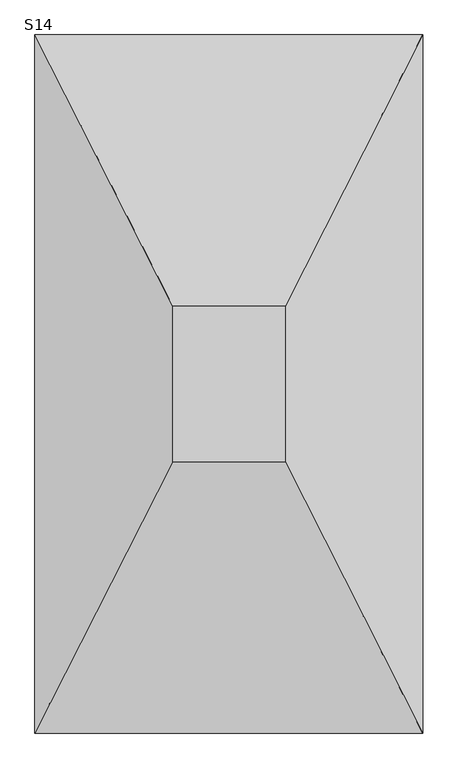
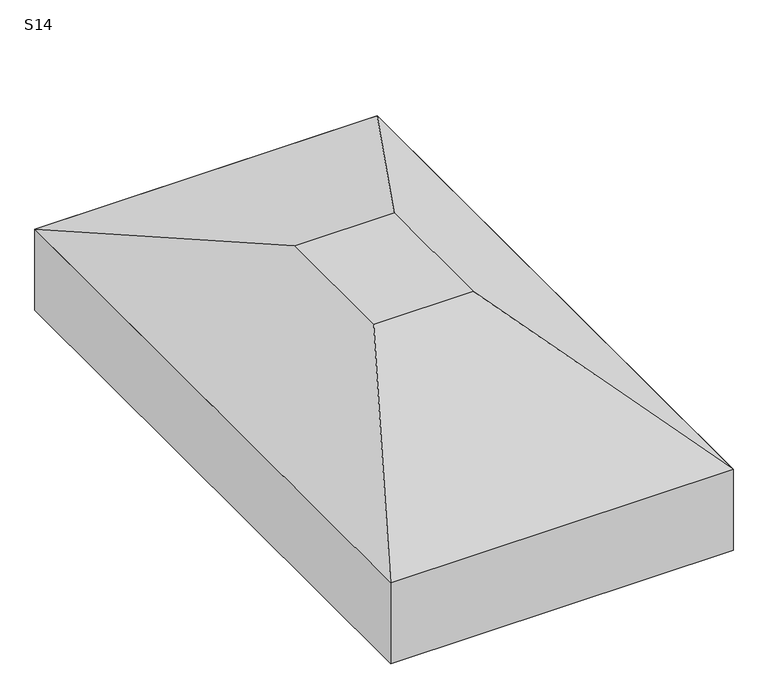
"""IFC4 building model written with IfcOpenShell, lengths in millimetres: fastener geometry, TQS - Sapata : S14."""

from ifc_helpers import new_model, si_unit, frame, origin, place, context, project, spatial, polyline, outline, extrude, faceted_brep, source, transform, mapped, element, save


def s14_8166d2be(model_context):
    return source(origin(), model_context, "Body", "SolidModel", [
        faceted_brep([(-55.0, 0.0, 0.0), (-345.0, 0.0, 0.0), (-345.0, -400.0, 0.0), (-55.0, -400.0, 0.0), (300.0, 700.0, -250.0), (300.0, -1100.0, -250.0), (-700.0, -1100.0, -250.0), (-700.0, 700.0, -250.0)], [[[0, 1, 2, 3]], [[4, 5, 6, 7]], [[4, 7, 1, 0]], [[7, 6, 2, 1]], [[6, 5, 3, 2]], [[5, 4, 0, 3]]]),
        extrude(outline(polyline([(300.0, 700.0), (300.0, -1100.0), (-700.0, -1100.0), (-700.0, 700.0), (300.0, 700.0)])), frame((0.0, 0.0, -500.0), z_axis=(0.0, 0.0, 1.0), x_axis=(1.0, 0.0, 0.0)), (0.0, 0.0, 1.0), 250.0),
    ])


if __name__ == "__main__":
    model = new_model("IFC4")
    model_context = context("Model", 3, world=origin())
    ifc_project = project(units=[si_unit("LENGTHUNIT", "METRE", prefix="MILLI")], contexts=[model_context])
    site = spatial("IfcSite", under=ifc_project)
    building = spatial("IfcBuilding", under=site)
    placement = place(None, origin())
    s14_shape = s14_8166d2be(model_context)
    element("IfcFastener", 1, ObjectType="TQS - Sapata : S14", at=placement, inside=building, context=model_context, shape_type="MappedRepresentation", body=[
        mapped(s14_shape, transform((0.0, 0.0, 0.0), x_axis=(1.0, 0.0, 0.0), y_axis=(0.0, 1.0, 0.0), z_axis=(0.0, 0.0, 1.0))),
    ])
    save(model, "model.ifc")

# Revit data of these elements
# Type "TQS - Sapata : S14"
#   TY = 0.40 m
#   TX = 0.29 m
#   HS = 0.50 m
#   H0 = 0.25 m
#   EXCYABS = 0.90 m
#   EXCY = 0.00 m
#   EXCXABS = 0.50 m
#   EXCX = 0.00 m
#   DIMY = 1.80 m
#   DIMX = 1.00 m
#   Material estrutural = Concreto - Concreto concretado no local
#   Width = 0
#   Length = 0
# Element 1 (IfcFastener, "TQS - Sapata : S14")
#   Materials on its faces: "Concreto - Concreto concretado no local"
# Materials
#   "Concreto - Concreto concretado no local": class "Concreto", colour RGB 192 192 192, transparency 0
